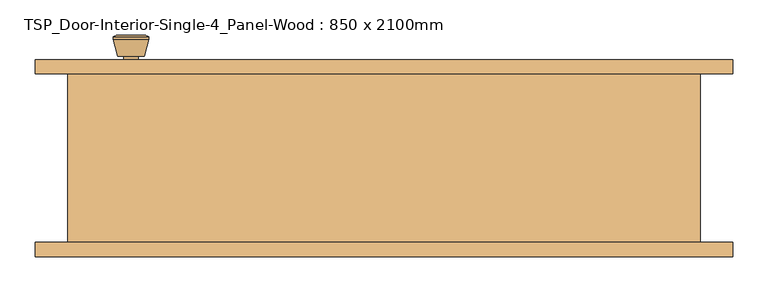
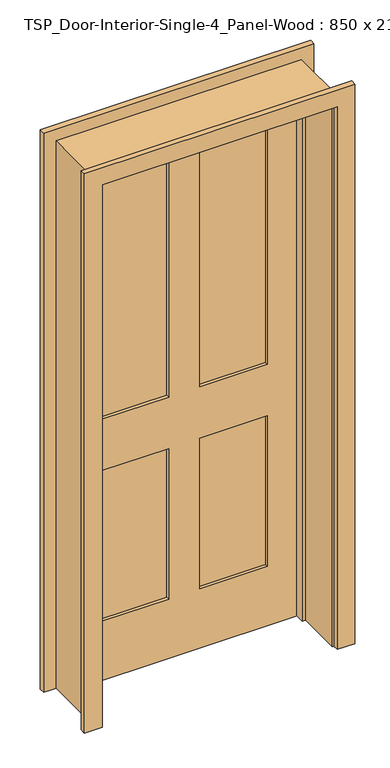
"""IFC4 building model written with IfcOpenShell, lengths in millimetres: door geometry, TSP_Door-Interior-Single-4_Panel-Wood : 850 x 2100mm."""

from ifc_helpers import new_model, si_unit, point, frame, frame_2d, origin, place, context, project, spatial, polyline, circle_curve, trimmed, segment, composite_curve, outline, extrude, faceted_brep, source, transform, mapped, element, save
from ifc_brep_helpers import plane_surface, cylinder_surface, revolved_surface, advanced_brep


def tsp_door_interior_single_4_panel_wood_850_x_2100mm_b606be2f(model_context):
    return source(origin(), model_context, "Body", "SolidModel", [
        advanced_brep(
        [(-360.0, 75.825, 914.4), (-350.0, 75.825, 914.4), (-370.0, 75.825, 914.4), (-339.5241324, 26.825, 914.4), (-360.0, 26.825, 914.4), (-380.4758676, 26.825, 914.4), (-335.0, 28.6528681, 914.4), (-385.0, 28.6528681, 914.4), (-335.0, 32.1165463, 914.4), (-385.0, 32.1165463, 914.4), (-341.363764, 56.825, 914.4), (-378.636236, 56.825, 914.4), (-350.0, 56.825, 914.4), (-370.0, 56.825, 914.4)],
        [
            (0, 1),
            (1, 2, circle_curve(frame((-360.0, 75.825, 914.4), z_axis=(0.0, 1.0, 0.0), x_axis=(-1.0, 0.0, 0.0)), 10.0)),
            (2, 0),
            (2, 1, circle_curve(frame((-360.0, 75.825, 914.4), z_axis=(0.0, 1.0, 0.0), x_axis=(-1.0, 0.0, 0.0)), 10.0)),
            (3, 4),
            (4, 5),
            (5, 3, circle_curve(frame((-360.0, 26.825, 914.4), z_axis=(0.0, -1.0, 0.0), x_axis=(-1.0, 0.0, 0.0)), 20.4758676)),
            (3, 5, circle_curve(frame((-360.0, 26.825, 914.4), z_axis=(0.0, -1.0, 0.0), x_axis=(-1.0, 0.0, 0.0)), 20.4758676)),
            (6, 3),
            (5, 7),
            (7, 6, circle_curve(frame((-360.0, 28.6528681, 914.4), z_axis=(0.0, -1.0, 0.0), x_axis=(-1.0, 0.0, 0.0)), 25.0)),
            (6, 7, circle_curve(frame((-360.0, 28.6528681, 914.4), z_axis=(0.0, -1.0, 0.0), x_axis=(-1.0, 0.0, 0.0)), 25.0)),
            (8, 6),
            (7, 9),
            (9, 8, circle_curve(frame((-360.0, 32.1165463, 914.4), z_axis=(0.0, -1.0, 0.0), x_axis=(-1.0, 0.0, 0.0)), 25.0)),
            (8, 9, circle_curve(frame((-360.0, 32.1165463, 914.4), z_axis=(0.0, -1.0, 0.0), x_axis=(-1.0, 0.0, 0.0)), 25.0)),
            (10, 8),
            (9, 11),
            (11, 10, circle_curve(frame((-360.0, 56.825, 914.4), z_axis=(0.0, -1.0, 0.0), x_axis=(-1.0, 0.0, 0.0)), 18.636236)),
            (10, 11, circle_curve(frame((-360.0, 56.825, 914.4), z_axis=(0.0, -1.0, 0.0), x_axis=(-1.0, 0.0, 0.0)), 18.636236)),
            (12, 10),
            (11, 13),
            (13, 12, circle_curve(frame((-360.0, 56.825, 914.4), z_axis=(0.0, -1.0, 0.0), x_axis=(-1.0, 0.0, 0.0)), 10.0)),
            (12, 13, circle_curve(frame((-360.0, 56.825, 914.4), z_axis=(0.0, -1.0, 0.0), x_axis=(-1.0, 0.0, 0.0)), 10.0)),
            (1, 12),
            (13, 2),
        ],
        [
            plane_surface(frame((-360.0, 75.825, 914.4), z_axis=(0.0, 1.0, 0.0), x_axis=(-1.0, 0.0, 0.0))),
            plane_surface(frame((-360.0, 26.825, 914.4), z_axis=(0.0, -1.0, 0.0), x_axis=(-1.0, 0.0, 0.0))),
            revolved_surface(polyline([(-380.4758676, 26.825, 914.4), (-385.0, 28.6528681, 914.4)]), (-360.0, 75.825, 914.4), (0.0, 1.0, 0.0)),
            cylinder_surface(frame((-360.0, 75.825, 914.4), z_axis=(0.0, 1.0, 0.0), x_axis=(-1.0, 0.0, 0.0)), 25.0),
            revolved_surface(polyline([(-385.0, 32.1165463, 914.4), (-378.636236, 56.825, 914.4)]), (-360.0, 75.825, 914.4), (0.0, 1.0, 0.0)),
            plane_surface(frame((-360.0, 56.825, 914.4), z_axis=(0.0, 1.0, 0.0), x_axis=(-1.0, 0.0, 0.0))),
            cylinder_surface(frame((-360.0, 75.825, 914.4), z_axis=(0.0, 1.0, 0.0), x_axis=(-1.0, 0.0, 0.0)), 10.0),
        ],
        [
            (0, [[1, 2, 3]]),
            (0, [[-3, 4, -1]]),
            (1, [[5, 6, 7]]),
            (1, [[-6, -5, 8]]),
            (2, [[9, -7, 10, 11]]),
            (2, [[-10, -8, -9, 12]]),
            (3, [[13, -11, 14, 15]]),
            (3, [[-14, -12, -13, 16]]),
            (4, [[17, -15, 18, 19]]),
            (4, [[-18, -16, -17, 20]]),
            (5, [[21, -19, 22, 23]]),
            (5, [[-22, -20, -21, 24]]),
            (6, [[25, -23, 26, -2]]),
            (6, [[-26, -24, -25, -4]]),
        ],
    ),
        extrude(outline(composite_curve([segment(trimmed(circle_curve(frame_2d((914.4, -360.0)), 30.0), [point((914.4, -390.0))], [point((914.4, -330.0))], False, "CARTESIAN"), True, "CONTINUOUS"), segment(trimmed(circle_curve(frame_2d((914.4, -360.0)), 30.0), [point((914.4, -330.0))], [point((914.4, -390.0))], False, "CARTESIAN"), True, "CONTINUOUS")], self_intersect=False)), frame((0.0, 75.825, 0.0), z_axis=(0.0, 1.0, 0.0), x_axis=(0.0, 0.0, 1.0)), (0.0, 0.0, 1.0), 6.0),
        advanced_brep(
        [(-360.0, 122.825, 914.4), (-370.0, 122.825, 914.4), (-350.0, 122.825, 914.4), (-339.5241324, 171.825, 914.4), (-380.4758676, 171.825, 914.4), (-360.0, 171.825, 914.4), (-335.0, 169.9971319, 914.4), (-385.0, 169.9971319, 914.4), (-335.0, 166.5334537, 914.4), (-385.0, 166.5334537, 914.4), (-341.363764, 141.825, 914.4), (-378.636236, 141.825, 914.4), (-350.0, 141.825, 914.4), (-370.0, 141.825, 914.4)],
        [
            (0, 1),
            (1, 2, circle_curve(frame((-360.0, 122.825, 914.4), z_axis=(0.0, -1.0, 0.0), x_axis=(-1.0, 0.0, 0.0)), 10.0)),
            (2, 0),
            (2, 1, circle_curve(frame((-360.0, 122.825, 914.4), z_axis=(0.0, -1.0, 0.0), x_axis=(-1.0, 0.0, 0.0)), 10.0)),
            (3, 4, circle_curve(frame((-360.0, 171.825, 914.4), z_axis=(0.0, 1.0, 0.0), x_axis=(-1.0, 0.0, 0.0)), 20.4758676)),
            (4, 5),
            (5, 3),
            (4, 3, circle_curve(frame((-360.0, 171.825, 914.4), z_axis=(0.0, 1.0, 0.0), x_axis=(-1.0, 0.0, 0.0)), 20.4758676)),
            (6, 7, circle_curve(frame((-360.0, 169.9971319, 914.4), z_axis=(0.0, 1.0, 0.0), x_axis=(-1.0, 0.0, 0.0)), 25.0)),
            (7, 4),
            (3, 6),
            (7, 6, circle_curve(frame((-360.0, 169.9971319, 914.4), z_axis=(0.0, 1.0, 0.0), x_axis=(-1.0, 0.0, 0.0)), 25.0)),
            (8, 9, circle_curve(frame((-360.0, 166.5334537, 914.4), z_axis=(0.0, 1.0, 0.0), x_axis=(-1.0, 0.0, 0.0)), 25.0)),
            (9, 7),
            (6, 8),
            (9, 8, circle_curve(frame((-360.0, 166.5334537, 914.4), z_axis=(0.0, 1.0, 0.0), x_axis=(-1.0, 0.0, 0.0)), 25.0)),
            (10, 11, circle_curve(frame((-360.0, 141.825, 914.4), z_axis=(0.0, 1.0, 0.0), x_axis=(-1.0, 0.0, 0.0)), 18.636236)),
            (11, 9),
            (8, 10),
            (11, 10, circle_curve(frame((-360.0, 141.825, 914.4), z_axis=(0.0, 1.0, 0.0), x_axis=(-1.0, 0.0, 0.0)), 18.636236)),
            (12, 13, circle_curve(frame((-360.0, 141.825, 914.4), z_axis=(0.0, 1.0, 0.0), x_axis=(-1.0, 0.0, 0.0)), 10.0)),
            (13, 11),
            (10, 12),
            (13, 12, circle_curve(frame((-360.0, 141.825, 914.4), z_axis=(0.0, 1.0, 0.0), x_axis=(-1.0, 0.0, 0.0)), 10.0)),
            (1, 13),
            (12, 2),
        ],
        [
            plane_surface(frame((-360.0, 122.825, 914.4), z_axis=(0.0, -1.0, 0.0), x_axis=(-1.0, 0.0, 0.0))),
            plane_surface(frame((-360.0, 171.825, 914.4), z_axis=(0.0, 1.0, 0.0), x_axis=(-1.0, 0.0, 0.0))),
            revolved_surface(polyline([(-380.4758676, 171.825, 914.4), (-385.0, 169.9971319, 914.4)]), (-360.0, 122.825, 914.4), (0.0, -1.0, 0.0)),
            cylinder_surface(frame((-360.0, 122.825, 914.4), z_axis=(0.0, -1.0, 0.0), x_axis=(-1.0, 0.0, 0.0)), 25.0),
            revolved_surface(polyline([(-385.0, 166.5334537, 914.4), (-378.636236, 141.825, 914.4)]), (-360.0, 122.825, 914.4), (0.0, -1.0, 0.0)),
            plane_surface(frame((-360.0, 141.825, 914.4), z_axis=(0.0, -1.0, 0.0), x_axis=(-1.0, 0.0, 0.0))),
            cylinder_surface(frame((-360.0, 122.825, 914.4), z_axis=(0.0, -1.0, 0.0), x_axis=(-1.0, 0.0, 0.0)), 10.0),
        ],
        [
            (0, [[1, 2, 3]]),
            (0, [[-3, 4, -1]]),
            (1, [[5, 6, 7]]),
            (1, [[8, -7, -6]]),
            (2, [[9, 10, -5, 11]]),
            (2, [[12, -11, -8, -10]]),
            (3, [[13, 14, -9, 15]]),
            (3, [[16, -15, -12, -14]]),
            (4, [[17, 18, -13, 19]]),
            (4, [[20, -19, -16, -18]]),
            (5, [[21, 22, -17, 23]]),
            (5, [[24, -23, -20, -22]]),
            (6, [[-2, 25, -21, 26]]),
            (6, [[-4, -26, -24, -25]]),
        ],
    ),
        extrude(outline(composite_curve([segment(trimmed(circle_curve(frame_2d((914.4, -360.0)), 30.0), [point((914.4, -390.0))], [point((914.4, -330.0))], False, "CARTESIAN"), True, "CONTINUOUS"), segment(trimmed(circle_curve(frame_2d((914.4, -360.0)), 30.0), [point((914.4, -330.0))], [point((914.4, -390.0))], False, "CARTESIAN"), True, "CONTINUOUS")], self_intersect=False)), frame((0.0, 116.825, 0.0), z_axis=(0.0, 1.0, 0.0), x_axis=(0.0, 0.0, 1.0)), (0.0, 0.0, 1.0), 6.0),
        faceted_brep([(450.0, 116.825, 0.0), (450.0, -123.175, 0.0), (425.0, -123.175, 0.0), (425.0, 46.9, 0.0), (412.3, 46.9, 0.0), (412.3, 81.825, 0.0), (425.0, 81.825, 0.0), (425.0, 116.825, 0.0), (450.0, 116.825, 2125.0), (450.0, -123.175, 2125.0), (-450.0, -123.175, 2125.0), (-450.0, -123.175, 0.0), (-425.0, -123.175, 0.0), (-425.0, -123.175, 2100.0), (425.0, -123.175, 2100.0), (425.0, 46.9, 2100.0), (-425.0, 46.9, 2100.0), (-425.0, 46.9, 0.0), (-412.3, 46.9, 0.0), (-412.3, 46.9, 2087.3), (412.3, 46.9, 2087.3), (412.3, 81.825, 2087.3), (-412.3, 81.825, 2087.3), (-412.3, 81.825, 0.0), (-425.0, 81.825, 0.0), (-425.0, 81.825, 2100.0), (425.0, 81.825, 2100.0), (425.0, 116.825, 2100.0), (-425.0, 116.825, 2100.0), (-425.0, 116.825, 0.0), (-450.0, 116.825, 0.0), (-450.0, 116.825, 2125.0)], [[[0, 1, 2, 3, 4, 5, 6, 7]], [[1, 0, 8, 9]], [[2, 1, 9, 10, 11, 12, 13, 14]], [[3, 2, 14, 15]], [[4, 3, 15, 16, 17, 18, 19, 20]], [[5, 4, 20, 21]], [[6, 5, 21, 22, 23, 24, 25, 26]], [[7, 6, 26, 27]], [[0, 7, 27, 28, 29, 30, 31, 8]], [[9, 8, 31, 10]], [[15, 14, 13, 16]], [[21, 20, 19, 22]], [[27, 26, 25, 28]], [[30, 29, 24, 23, 18, 17, 12, 11]], [[10, 31, 30, 11]], [[16, 13, 12, 17]], [[22, 19, 18, 23]], [[28, 25, 24, 29]]]),
        extrude(outline(polyline([(2100.0, -425.0), (0.0, -425.0), (0.0, 425.0), (2100.0, 425.0), (2100.0, -425.0)]), holes=[polyline([(1980.0, 57.5), (1980.0, 305.0), (1014.4, 305.0), (1014.4, 57.5), (1980.0, 57.5)]), polyline([(1014.4, -57.5), (1014.4, -305.0), (1980.0, -305.0), (1980.0, -57.5), (1014.4, -57.5)]), polyline([(814.4, 57.5), (814.4, 305.0), (230.0, 305.0), (230.0, 57.5), (814.4, 57.5)]), polyline([(230.0, -57.5), (230.0, -305.0), (814.4, -305.0), (814.4, -57.5), (230.0, -57.5)])]), frame((0.0, 81.825, 0.0), z_axis=(0.0, 1.0, 0.0), x_axis=(0.0, 0.0, 1.0)), (0.0, 0.0, 1.0), 35.0),
        extrude(outline(polyline([(305.0, 93.4916667), (57.5, 93.4916667), (57.5, 105.1583333), (305.0, 105.1583333), (305.0, 93.4916667)])), frame((0.0, 0.0, 1014.4), z_axis=(0.0, 0.0, 1.0), x_axis=(1.0, 0.0, 0.0)), (0.0, 0.0, 1.0), 965.6),
        extrude(outline(polyline([(-57.5, 93.4916667), (-305.0, 93.4916667), (-305.0, 105.1583333), (-57.5, 105.1583333), (-57.5, 93.4916667)])), frame((0.0, 0.0, 1014.4), z_axis=(0.0, 0.0, 1.0), x_axis=(1.0, 0.0, 0.0)), (0.0, 0.0, 1.0), 965.6),
        extrude(outline(polyline([(305.0, 93.4916667), (57.5, 93.4916667), (57.5, 105.1583333), (305.0, 105.1583333), (305.0, 93.4916667)])), frame((0.0, 0.0, 230.0), z_axis=(0.0, 0.0, 1.0), x_axis=(1.0, 0.0, 0.0)), (0.0, 0.0, 1.0), 584.4),
        extrude(outline(polyline([(-57.5, 93.4916667), (-305.0, 93.4916667), (-305.0, 105.1583333), (-57.5, 105.1583333), (-57.5, 93.4916667)])), frame((0.0, 0.0, 230.0), z_axis=(0.0, 0.0, 1.0), x_axis=(1.0, 0.0, 0.0)), (0.0, 0.0, 1.0), 584.4),
        extrude(outline(polyline([(0.0, 431.35), (0.0, 496.35), (2171.35, 496.35), (2171.35, -496.35), (0.0, -496.35), (0.0, -431.35), (2106.35, -431.35), (2106.35, 431.35), (0.0, 431.35)])), frame((0.0, 116.825, 0.0), z_axis=(0.0, 1.0, 0.0), x_axis=(0.0, 0.0, 1.0)), (0.0, 0.0, 1.0), 20.0),
        extrude(outline(polyline([(0.0, 431.35), (0.0, 496.35), (2171.35, 496.35), (2171.35, -496.35), (0.0, -496.35), (0.0, -431.35), (2106.35, -431.35), (2106.35, 431.35), (0.0, 431.35)])), frame((0.0, -143.175, 0.0), z_axis=(0.0, 1.0, 0.0), x_axis=(0.0, 0.0, 1.0)), (0.0, 0.0, 1.0), 20.0),
    ])


if __name__ == "__main__":
    model = new_model("IFC4")
    model_context = context("Model", 3, world=origin())
    ifc_project = project(units=[si_unit("LENGTHUNIT", "METRE", prefix="MILLI")], contexts=[model_context])
    site = spatial("IfcSite", under=ifc_project)
    building = spatial("IfcBuilding", under=site)
    placement = place(None, origin())
    tsp_door_interior_single_4_panel_wood_850_x_2100mm_shape = tsp_door_interior_single_4_panel_wood_850_x_2100mm_b606be2f(model_context)
    element("IfcDoor", 1, ObjectType="TSP_Door-Interior-Single-4_Panel-Wood : 850 x 2100mm", at=placement, inside=building, context=model_context, shape_type="MappedRepresentation", body=[
        mapped(tsp_door_interior_single_4_panel_wood_850_x_2100mm_shape, transform((0.0, 0.0, 0.0), x_axis=(1.0, 0.0, 0.0), y_axis=(0.0, 1.0, 0.0), z_axis=(0.0, 0.0, 1.0))),
    ])
    save(model, "model.ifc")

# Revit data of these elements
# Type "TSP_Door-Interior-Single-4_Panel-Wood : 850 x 2100mm"
#   Model = "TSP_DOOR02W"
#   Type Mark = "243"
#   Assembly Code = "C1020300"
#   Analytic Construction = "Wooden"
#   Top Rail = 120 mm
#   Thickness = 35 mm
#   Thermal Resistance (R) = 0.455703 (m²·K)/W
#   Swing Angle [instance default] = 90.00°
#   Stiles = 120 mm
#   Rough Width = 900 mm
#   Rough Height = 2125 mm
#   Mullion = 115 mm
#   Lock Rail = 200 mm
#   Height = 2100 mm
#   Width = 850 mm
#   Heat Transfer Coefficient (U) = 2.19465 W/(m²·K)
#   Bottom Rail = 230 mm
#   Define Thermal Properties by = 1
#   Trim Material = Cherry
#   Panel Material = Cherry
#   Frame Material = Cherry
#   Door Handle Material = Aluminum
#   Visual Light Transmittance = 0
#   Solar Heat Gain Coefficient = 0
#   Wall Closure = (empty or 0)
#   Function = (empty or 0)
# Element 1 (IfcDoor, "TSP_Door-Interior-Single-4_Panel-Wood : 850 x 2100mm")
#   Materials on its faces: "Cherry", "Aluminum"
# Materials
#   "Cherry": class "Wood", colour RGB 226 177 128, transparency 0, Description = "Prunus Serotina", Cost = 0
#   "Aluminum": class "Metal", colour RGB 247 247 247, transparency 0, Description = "Aluminum 6061", Cost = 0
